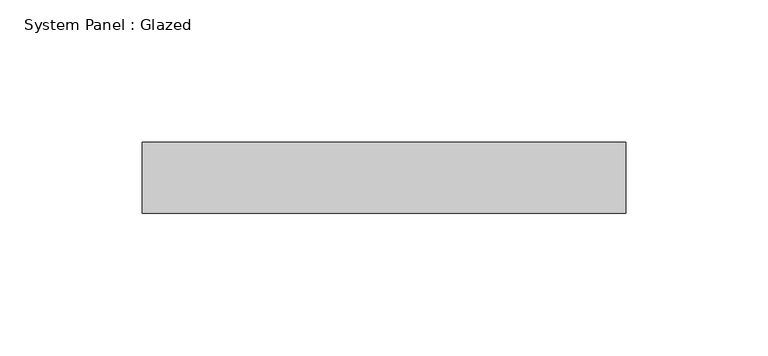
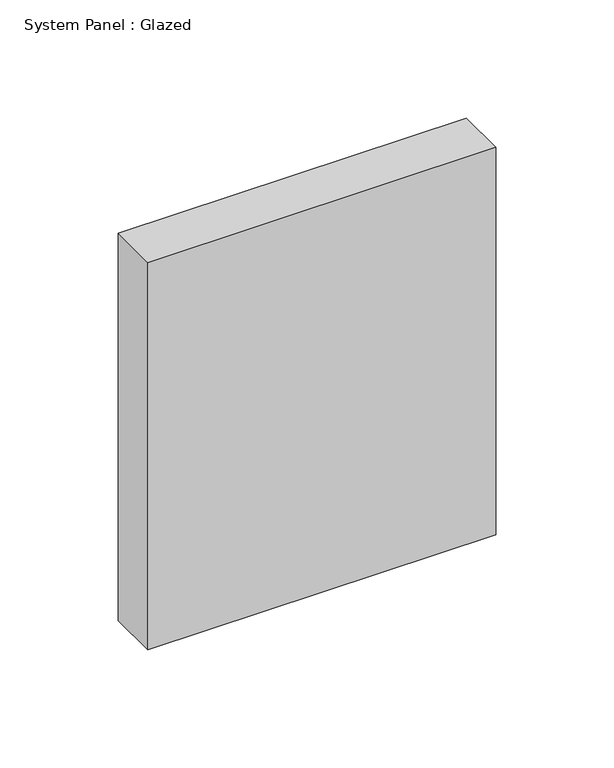
"""IFC4 building model written with IfcOpenShell, lengths in millimetres: plate geometry, System Panel : Glazed."""

from ifc_helpers import new_model, si_unit, origin, origin_with_axes, place, context, project, spatial, polyline, outline, extrude, source, transform, mapped, element, save


def system_panel_glazed_1ea8d406(model_context):
    return source(origin(), model_context, "Body", "SweptSolid", [
        extrude(outline(polyline([(85.0, 24.5), (-85.0, 24.5), (-85.0, 49.5), (85.0, 49.5), (85.0, 24.5)])), origin_with_axes(), (0.0, 0.0, 1.0), 200.0),
    ])


if __name__ == "__main__":
    model = new_model("IFC4")
    model_context = context("Model", 3, world=origin())
    ifc_project = project(units=[si_unit("LENGTHUNIT", "METRE", prefix="MILLI")], contexts=[model_context])
    site = spatial("IfcSite", under=ifc_project)
    building = spatial("IfcBuilding", under=site)
    placement = place(None, origin())
    system_panel_glazed_shape = system_panel_glazed_1ea8d406(model_context)
    element("IfcPlate", 1, ObjectType="System Panel : Glazed", at=placement, inside=building, context=model_context, shape_type="MappedRepresentation", body=[
        mapped(system_panel_glazed_shape, transform((0.0, 0.0, 0.0), x_axis=(1.0, 0.0, 0.0), y_axis=(0.0, 1.0, 0.0), z_axis=(0.0, 0.0, 1.0))),
    ])
    save(model, "model.ifc")

# Revit data of these elements
# Element 1 (IfcPlate, "System Panel : Glazed")
#   Materials on its faces: "Glass"
# Materials
#   "Glass": class "Glass", colour RGB 218 227 224, transparency 0.85, Description = "Soda Lime Glass", Cost = 0
